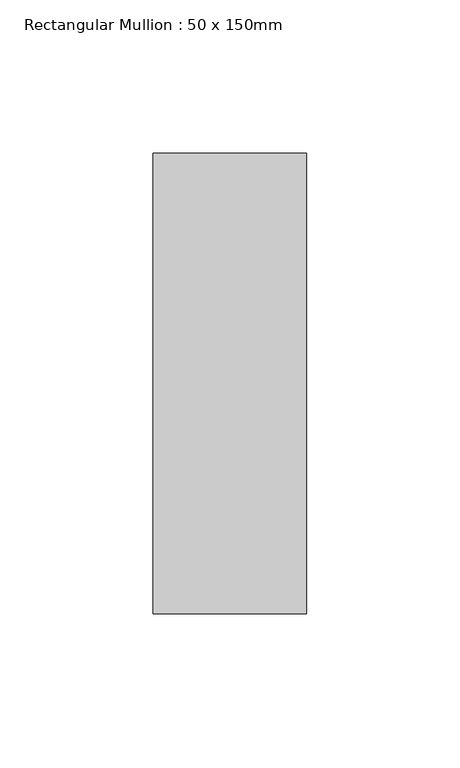
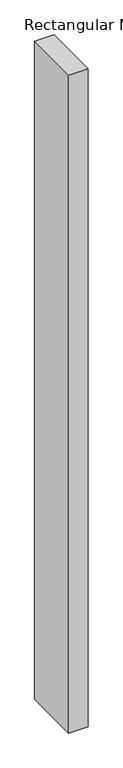
"""IFC4 building model written with IfcOpenShell, lengths in millimetres: member geometry, Rectangular Mullion : 50 x 150mm."""

from ifc_helpers import new_model, si_unit, frame, origin, place, context, project, spatial, polyline, outline, extrude, source, transform, mapped, element, save


def rectangular_mullion_50_x_150mm_1e81bce4(model_context):
    return source(origin(), model_context, "Body", "SweptSolid", [
        extrude(outline(polyline([(0.0, 75.0), (0.0, -75.0), (-50.0, -75.0), (-50.0, 75.0), (0.0, 75.0)])), frame((0.0, 0.0, -1775.8970067), z_axis=(0.0, 0.0, 1.0), x_axis=(1.0, 0.0, 0.0)), (0.0, 0.0, 1.0), 1775.8970067),
    ])


if __name__ == "__main__":
    model = new_model("IFC4")
    model_context = context("Model", 3, world=origin())
    ifc_project = project(units=[si_unit("LENGTHUNIT", "METRE", prefix="MILLI")], contexts=[model_context])
    site = spatial("IfcSite", under=ifc_project)
    building = spatial("IfcBuilding", under=site)
    placement = place(None, origin())
    rectangular_mullion_50_x_150mm_shape = rectangular_mullion_50_x_150mm_1e81bce4(model_context)
    element("IfcMember", 1, ObjectType="Rectangular Mullion : 50 x 150mm", at=placement, inside=building, context=model_context, shape_type="MappedRepresentation", body=[
        mapped(rectangular_mullion_50_x_150mm_shape, transform((0.0, 0.0, 0.0), x_axis=(1.0, 0.0, 0.0), y_axis=(0.0, 1.0, 0.0), z_axis=(0.0, 0.0, 1.0))),
    ])
    save(model, "model.ifc")

# Revit data of these elements
# Project information
#   Document_Suitability_Code = "A1"
#   Document_Suitability_Description = "Coordination"
#   Project Status = "Project Status"
#   Client Name = "Revit Project"
#   Project Address = "Limerick Institute of Technology"
#   Project Name = "Commercial Units"
#   Project Number = "RARC02"
# Type "Rectangular Mullion : 50 x 150mm"
#   Keynote = "H11"
#   built-in parameter 1007304 = 0.492126 (stored number, unit not read)
#   built-in parameter 1007301 = 0.082021 (stored number, unit not read)
#   built-in parameter 1007300 = 0.082021 (stored number, unit not read)
# Element 1 (IfcMember, "Rectangular Mullion : 50 x 150mm")
#   Materials on its faces: "Aluminium"
# Materials
#   "Aluminium": class "Metal", colour RGB 247 247 247, transparency 0, Description = "Aluminium 6061", Cost = 0
